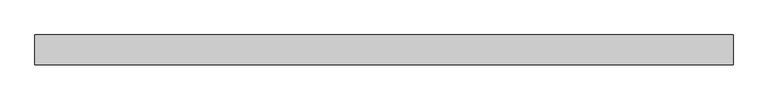
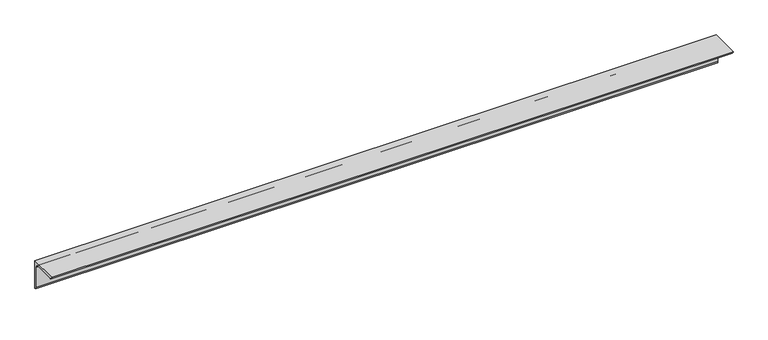
"""IFC4 building model written with IfcOpenShell, lengths in millimetres: beam geometry, 0912_Steel Framing_L-KSD3502 : H_SB_AR_S04_L-130x130x12_KBR1."""

from ifc_helpers import new_model, si_unit, point, frame, frame_2d, origin, place, context, project, spatial, polyline, circle_curve, trimmed, segment, composite_curve, outline, extrude, source, transform, mapped, element, save


def beam_d8285e93(model_context):
    return source(origin(), model_context, "Body", "SweptSolid", [
        extrude(outline(composite_curve([segment(polyline([(36.4, 36.4), (36.4, -93.6)]), True, "CONTINUOUS"), segment(trimmed(circle_curve(frame_2d((36.4, -81.6)), 12.0), [point((36.4, -93.6))], [point((24.4, -81.6))], False, "CARTESIAN"), True, "CONTINUOUS"), segment(polyline([(24.4, -81.6), (24.4, 12.4)]), True, "CONTINUOUS"), segment(trimmed(circle_curve(frame_2d((12.4, 12.4)), 12.0), [point((24.4, 12.4))], [point((12.4, 24.4))], True, "CARTESIAN"), True, "CONTINUOUS"), segment(polyline([(12.4, 24.4), (-81.6, 24.4)]), True, "CONTINUOUS"), segment(trimmed(circle_curve(frame_2d((-81.6, 36.4)), 12.0), [point((-81.6, 24.4))], [point((-93.6, 36.4))], False, "CARTESIAN"), True, "CONTINUOUS"), segment(polyline([(-93.6, 36.4), (36.4, 36.4)]), True, "CONTINUOUS")], self_intersect=False)), frame((-1519.4237854, 0.0, 0.0), z_axis=(1.0, 0.0, 0.0), x_axis=(0.0, 1.0, 0.0)), (0.0, 0.0, 1.0), 3039.6020843),
    ])


if __name__ == "__main__":
    model = new_model("IFC4")
    model_context = context("Model", 3, world=origin())
    ifc_project = project(units=[si_unit("LENGTHUNIT", "METRE", prefix="MILLI")], contexts=[model_context])
    site = spatial("IfcSite", under=ifc_project)
    building = spatial("IfcBuilding", under=site)
    placement = place(None, origin())
    beam_shape = beam_d8285e93(model_context)
    element("IfcBeam", 1, ObjectType="0912_Steel Framing_L-KSD3502 : H_SB_AR_S04_L-130x130x12_KBR1", at=placement, inside=building, context=model_context, shape_type="MappedRepresentation", body=[
        mapped(beam_shape, transform((0.0, 0.0, 0.0), x_axis=(1.0, 0.0, 0.0), y_axis=(0.0, 1.0, 0.0), z_axis=(0.0, 0.0, 1.0))),
    ])
    save(model, "model.ifc")

# Revit data of these elements
# Type "0912_Steel Framing_L-KSD3502 : H_SB_AR_S04_L-130x130x12_KBR1"
#   k = 25 mm
#   Perimeter = 0.52 m²/m
#   Nominal Weight = 23.40 kgf/m
#   Length [instance default] = 1000 mm
#   b = 130 mm
#   d = 130 mm
#   t = 12 mm
#   x = 36.4 mm
#   y = 36.4 mm
#   A = 2976.00 m²
#   Structural Material [instance default] = Steel, 45-345
# Element 1 (IfcBeam, "0912_Steel Framing_L-KSD3502 : H_SB_AR_S04_L-130x130x12_KBR1")
#   Structural Material = Steel ASTM A36
#   Materials on its faces: "Steel ASTM A36"
# Materials
#   "Steel, 45-345": class "Metal", colour RGB 189 187 185, transparency 0, Description = "Steel 345 MPa", Cost = 0
#   "Steel ASTM A36": class "Metal", colour RGB 199 199 199, transparency 0, Description = "Structural steel, ASTM A36 Grade B, mill finish", Cost = 0
